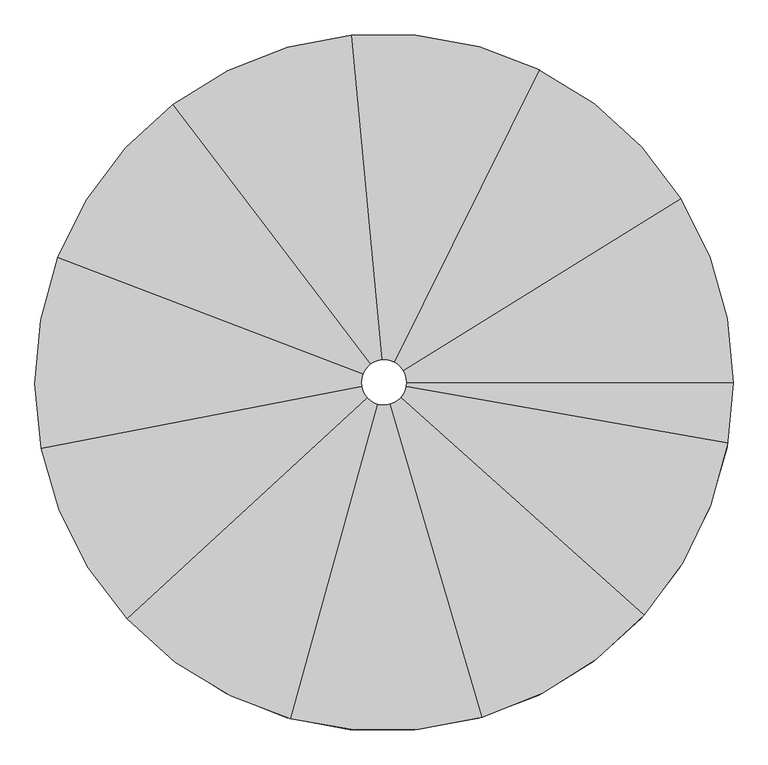
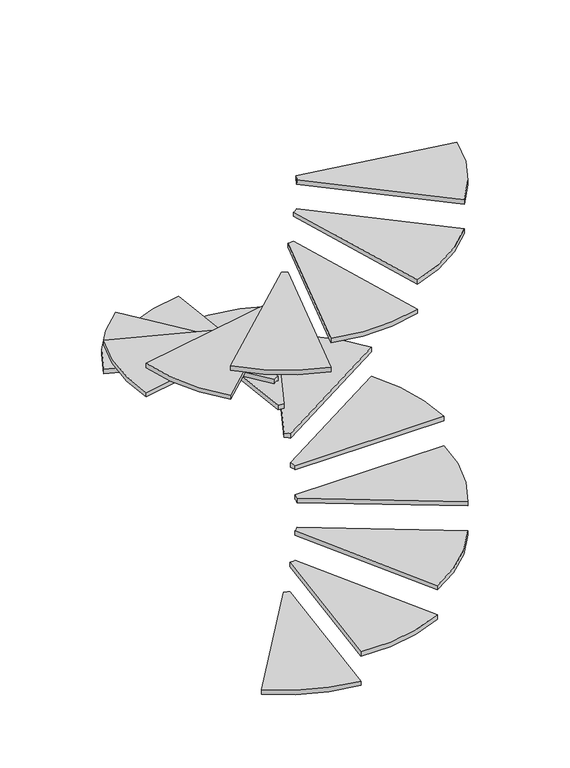
"""IFC4 building model written with IfcOpenShell, lengths in millimetres: stair flight geometry."""

from ifc_helpers import new_model, si_unit, point, frame, frame_2d, origin, place, context, project, spatial, polyline, circle_curve, trimmed, segment, composite_curve, outline, extrude, source, transform, mapped, element, save


def stair_flight_6586929f(model_context):
    return source(origin(), model_context, "Body", "SweptSolid", [
        extrude(outline(composite_curve([segment(polyline([(21449.895584, -2902.3142462), (21371.5931684, -3711.3337588)]), True, "CONTINUOUS"), segment(trimmed(circle_curve(frame_2d((21455.3703815, -2845.7487117)), 869.6298611), [point((21371.5931684, -3711.3337588))], [point((20927.7521934, -3537.0338502))], False, "CARTESIAN"), True, "CONTINUOUS"), segment(polyline([(20927.7521934, -3537.0338502), (21420.8908061, -2890.9238375)]), True, "CONTINUOUS"), segment(trimmed(circle_curve(frame_2d((21455.3703815, -2845.7487117)), 56.8298611), [point((21420.8908061, -2890.9238375))], [point((21449.895584, -2902.3142462))], True, "CARTESIAN"), True, "CONTINUOUS")], self_intersect=False)), frame((0.0, 0.0, 142.875), z_axis=(0.0, 0.0, 1.0), x_axis=(1.0, 0.0, 0.0)), (0.0, 0.0, 1.0), 25.4),
        extrude(outline(composite_curve([segment(polyline([(21480.5464095, -2896.6977129), (21840.6225241, -3625.387655)]), True, "CONTINUOUS"), segment(trimmed(circle_curve(frame_2d((21455.3703815, -2845.7487117)), 869.6298611), [point((21840.6225241, -3625.387655))], [point((21371.5931684, -3711.3337588))], False, "CARTESIAN"), True, "CONTINUOUS"), segment(polyline([(21371.5931684, -3711.3337588), (21449.895584, -2902.3142462)]), True, "CONTINUOUS"), segment(trimmed(circle_curve(frame_2d((21455.3703815, -2845.7487117)), 56.8298611), [point((21449.895584, -2902.3142462))], [point((21480.5464095, -2896.6977129))], True, "CARTESIAN"), True, "CONTINUOUS")], self_intersect=False)), frame((0.0, 0.0, 311.15), z_axis=(0.0, 0.0, 1.0), x_axis=(1.0, 0.0, 0.0)), (0.0, 0.0, 1.0), 25.4),
        extrude(outline(composite_curve([segment(polyline([(21503.6278333, -2875.7628992), (22193.8223212, -3305.0360161)]), True, "CONTINUOUS"), segment(trimmed(circle_curve(frame_2d((21455.3703815, -2845.7487117)), 869.6298611), [point((22193.8223212, -3305.0360161))], [point((21840.6225241, -3625.387655))], False, "CARTESIAN"), True, "CONTINUOUS"), segment(polyline([(21840.6225241, -3625.387655), (21480.5464095, -2896.6977129)]), True, "CONTINUOUS"), segment(trimmed(circle_curve(frame_2d((21455.3703815, -2845.7487117)), 56.8298611), [point((21480.5464095, -2896.6977129))], [point((21503.6278333, -2875.7628992))], True, "CARTESIAN"), True, "CONTINUOUS")], self_intersect=False)), frame((0.0, 0.0, 479.425), z_axis=(0.0, 0.0, 1.0), x_axis=(1.0, 0.0, 0.0)), (0.0, 0.0, 1.0), 25.4),
        extrude(outline(composite_curve([segment(polyline([(21512.2002156, -2845.8040472), (22324.9998303, -2846.5954743)]), True, "CONTINUOUS"), segment(trimmed(circle_curve(frame_2d((21455.3703815, -2845.7487117)), 869.6298611), [point((22324.9998303, -2846.5954743))], [point((22193.8223212, -3305.0360161))], False, "CARTESIAN"), True, "CONTINUOUS"), segment(polyline([(22193.8223212, -3305.0360161), (21503.6278333, -2875.7628992)]), True, "CONTINUOUS"), segment(trimmed(circle_curve(frame_2d((21455.3703815, -2845.7487117)), 56.8298611), [point((21503.6278333, -2875.7628992))], [point((21512.2002156, -2845.8040472))], True, "CARTESIAN"), True, "CONTINUOUS")], self_intersect=False)), frame((0.0, 0.0, 647.7), z_axis=(0.0, 0.0, 1.0), x_axis=(1.0, 0.0, 0.0)), (0.0, 0.0, 1.0), 25.4),
        extrude(outline(composite_curve([segment(polyline([(21503.6861917, -2815.828558), (22194.7153409, -2387.9003456)]), True, "CONTINUOUS"), segment(trimmed(circle_curve(frame_2d((21455.3703815, -2845.7487117)), 869.6298611), [point((22194.7153409, -2387.9003456))], [point((22324.9998303, -2846.5954743))], False, "CARTESIAN"), True, "CONTINUOUS"), segment(polyline([(22324.9998303, -2846.5954743), (21512.2002156, -2845.8040472)]), True, "CONTINUOUS"), segment(trimmed(circle_curve(frame_2d((21455.3703815, -2845.7487117)), 56.8298611), [point((21512.2002156, -2845.8040472))], [point((21503.6861917, -2815.828558))], True, "CARTESIAN"), True, "CONTINUOUS")], self_intersect=False)), frame((0.0, 0.0, 815.975), z_axis=(0.0, 0.0, 1.0), x_axis=(1.0, 0.0, 0.0)), (0.0, 0.0, 1.0), 25.4),
        extrude(outline(composite_curve([segment(polyline([(21480.6455803, -2794.8488351), (21842.140069, -2066.8614899)]), True, "CONTINUOUS"), segment(trimmed(circle_curve(frame_2d((21455.3703815, -2845.7487117)), 869.6298611), [point((21842.140069, -2066.8614899))], [point((22194.7153409, -2387.9003456))], False, "CARTESIAN"), True, "CONTINUOUS"), segment(polyline([(22194.7153409, -2387.9003456), (21503.6861917, -2815.828558)]), True, "CONTINUOUS"), segment(trimmed(circle_curve(frame_2d((21455.3703815, -2845.7487117)), 56.8298611), [point((21503.6861917, -2815.828558))], [point((21480.6455803, -2794.8488351))], True, "CARTESIAN"), True, "CONTINUOUS")], self_intersect=False)), frame((0.0, 0.0, 984.25), z_axis=(0.0, 0.0, 1.0), x_axis=(1.0, 0.0, 0.0)), (0.0, 0.0, 1.0), 25.4),
        extrude(outline(composite_curve([segment(polyline([(21450.0057506, -2789.1726227), (21373.2789748, -1980.0021574)]), True, "CONTINUOUS"), segment(trimmed(circle_curve(frame_2d((21455.3703815, -2845.7487117)), 869.6298611), [point((21373.2789748, -1980.0021574))], [point((21842.140069, -2066.8614899))], False, "CARTESIAN"), True, "CONTINUOUS"), segment(polyline([(21842.140069, -2066.8614899), (21480.6455803, -2794.8488351)]), True, "CONTINUOUS"), segment(trimmed(circle_curve(frame_2d((21455.3703815, -2845.7487117)), 56.8298611), [point((21480.6455803, -2794.8488351))], [point((21450.0057506, -2789.1726227))], True, "CARTESIAN"), True, "CONTINUOUS")], self_intersect=False)), frame((0.0, 0.0, 1152.525), z_axis=(0.0, 0.0, 1.0), x_axis=(1.0, 0.0, 0.0)), (0.0, 0.0, 1.0), 25.4),
        extrude(outline(composite_curve([segment(polyline([(21420.9788459, -2800.5065257), (20929.0994083, -2153.4373958)]), True, "CONTINUOUS"), segment(trimmed(circle_curve(frame_2d((21455.3703815, -2845.7487117)), 869.6298611), [point((20929.0994083, -2153.4373958))], [point((21373.2789748, -1980.0021574))], False, "CARTESIAN"), True, "CONTINUOUS"), segment(polyline([(21373.2789748, -1980.0021574), (21450.0057506, -2789.1726227)]), True, "CONTINUOUS"), segment(trimmed(circle_curve(frame_2d((21455.3703815, -2845.7487117)), 56.8298611), [point((21450.0057506, -2789.1726227))], [point((21420.9788459, -2800.5065257))], True, "CARTESIAN"), True, "CONTINUOUS")], self_intersect=False)), frame((0.0, 0.0, 1320.8), z_axis=(0.0, 0.0, 1.0), x_axis=(1.0, 0.0, 0.0)), (0.0, 0.0, 1.0), 25.4),
        extrude(outline(composite_curve([segment(polyline([(21402.292069, -2825.4429031), (20643.1479935, -2535.0223243)]), True, "CONTINUOUS"), segment(trimmed(circle_curve(frame_2d((21455.3703815, -2845.7487117)), 869.6298611), [point((20643.1479935, -2535.0223243))], [point((20929.0994083, -2153.4373958))], False, "CARTESIAN"), True, "CONTINUOUS"), segment(polyline([(20929.0994083, -2153.4373958), (21420.9788459, -2800.5065257)]), True, "CONTINUOUS"), segment(trimmed(circle_curve(frame_2d((21455.3703815, -2845.7487117)), 56.8298611), [point((21420.9788459, -2800.5065257))], [point((21402.292069, -2825.4429031))], True, "CARTESIAN"), True, "CONTINUOUS")], self_intersect=False)), frame((0.0, 0.0, 1489.075), z_axis=(0.0, 0.0, 1.0), x_axis=(1.0, 0.0, 0.0)), (0.0, 0.0, 1.0), 25.4),
        extrude(outline(composite_curve([segment(polyline([(21399.5637693, -2856.4844065), (20601.3986226, -3010.0299656)]), True, "CONTINUOUS"), segment(trimmed(circle_curve(frame_2d((21455.3703815, -2845.7487117)), 869.6298611), [point((20601.3986226, -3010.0299656))], [point((20643.1479935, -2535.0223243))], False, "CARTESIAN"), True, "CONTINUOUS"), segment(polyline([(20643.1479935, -2535.0223243), (21402.292069, -2825.4429031)]), True, "CONTINUOUS"), segment(trimmed(circle_curve(frame_2d((21455.3703815, -2845.7487117)), 56.8298611), [point((21402.292069, -2825.4429031))], [point((21399.5637693, -2856.4844065))], True, "CARTESIAN"), True, "CONTINUOUS")], self_intersect=False)), frame((0.0, 0.0, 1657.35), z_axis=(0.0, 0.0, 1.0), x_axis=(1.0, 0.0, 0.0)), (0.0, 0.0, 1.0), 25.4),
        extrude(outline(composite_curve([segment(polyline([(21413.6142347, -2884.2981257), (20816.4036234, -3435.6449546)]), True, "CONTINUOUS"), segment(trimmed(circle_curve(frame_2d((21455.3703815, -2845.7487117)), 869.6298611), [point((20816.4036234, -3435.6449546))], [point((20601.3986226, -3010.0299656))], False, "CARTESIAN"), True, "CONTINUOUS"), segment(polyline([(20601.3986226, -3010.0299656), (21399.5637693, -2856.4844065)]), True, "CONTINUOUS"), segment(trimmed(circle_curve(frame_2d((21455.3703815, -2845.7487117)), 56.8298611), [point((21399.5637693, -2856.4844065))], [point((21413.6142347, -2884.2981257))], True, "CARTESIAN"), True, "CONTINUOUS")], self_intersect=False)), frame((0.0, 0.0, 1825.625), z_axis=(0.0, 0.0, 1.0), x_axis=(1.0, 0.0, 0.0)), (0.0, 0.0, 1.0), 25.4),
        extrude(outline(composite_curve([segment(polyline([(21440.2190653, -2900.5216131), (21223.5197881, -3683.9022761)]), True, "CONTINUOUS"), segment(trimmed(circle_curve(frame_2d((21455.3703815, -2845.7487117)), 869.6298611), [point((21223.5197881, -3683.9022761))], [point((20816.4036234, -3435.6449546))], False, "CARTESIAN"), True, "CONTINUOUS"), segment(polyline([(20816.4036234, -3435.6449546), (21413.6142347, -2884.2981257)]), True, "CONTINUOUS"), segment(trimmed(circle_curve(frame_2d((21455.3703815, -2845.7487117)), 56.8298611), [point((21413.6142347, -2884.2981257))], [point((21440.2190653, -2900.5216131))], True, "CARTESIAN"), True, "CONTINUOUS")], self_intersect=False)), frame((0.0, 0.0, 1993.9), z_axis=(0.0, 0.0, 1.0), x_axis=(1.0, 0.0, 0.0)), (0.0, 0.0, 1.0), 25.4),
        extrude(outline(composite_curve([segment(polyline([(21471.3792768, -2900.2771298), (21700.3439412, -3680.1611099)]), True, "CONTINUOUS"), segment(trimmed(circle_curve(frame_2d((21455.3703815, -2845.7487117)), 869.6298611), [point((21700.3439412, -3680.1611099))], [point((21223.5197881, -3683.9022761))], False, "CARTESIAN"), True, "CONTINUOUS"), segment(polyline([(21223.5197881, -3683.9022761), (21440.2190653, -2900.5216131)]), True, "CONTINUOUS"), segment(trimmed(circle_curve(frame_2d((21455.3703815, -2845.7487117)), 56.8298611), [point((21440.2190653, -2900.5216131))], [point((21471.3792768, -2900.2771298))], True, "CARTESIAN"), True, "CONTINUOUS")], self_intersect=False)), frame((0.0, 0.0, 2162.175), z_axis=(0.0, 0.0, 1.0), x_axis=(1.0, 0.0, 0.0)), (0.0, 0.0, 1.0), 25.4),
        extrude(outline(composite_curve([segment(polyline([(21497.7262684, -2883.6381819), (22103.5145667, -3425.5462715)]), True, "CONTINUOUS"), segment(trimmed(circle_curve(frame_2d((21455.3703815, -2845.7487117)), 869.6298611), [point((22103.5145667, -3425.5462715))], [point((21700.3439412, -3680.1611099))], False, "CARTESIAN"), True, "CONTINUOUS"), segment(polyline([(21700.3439412, -3680.1611099), (21471.3792768, -2900.2771298)]), True, "CONTINUOUS"), segment(trimmed(circle_curve(frame_2d((21455.3703815, -2845.7487117)), 56.8298611), [point((21471.3792768, -2900.2771298))], [point((21497.7262684, -2883.6381819))], True, "CARTESIAN"), True, "CONTINUOUS")], self_intersect=False)), frame((0.0, 0.0, 2330.45), z_axis=(0.0, 0.0, 1.0), x_axis=(1.0, 0.0, 0.0)), (0.0, 0.0, 1.0), 25.4),
        extrude(outline(composite_curve([segment(polyline([(21511.3385776, -2855.6074205), (22311.8147515, -2996.6100265)]), True, "CONTINUOUS"), segment(trimmed(circle_curve(frame_2d((21455.3703815, -2845.7487117)), 869.6298611), [point((22311.8147515, -2996.6100265))], [point((22103.5145667, -3425.5462715))], False, "CARTESIAN"), True, "CONTINUOUS"), segment(polyline([(22103.5145667, -3425.5462715), (21497.7262684, -2883.6381819)]), True, "CONTINUOUS"), segment(trimmed(circle_curve(frame_2d((21455.3703815, -2845.7487117)), 56.8298611), [point((21497.7262684, -2883.6381819))], [point((21511.3385776, -2855.6074205))], True, "CARTESIAN"), True, "CONTINUOUS")], self_intersect=False)), frame((0.0, 0.0, 2498.725), z_axis=(0.0, 0.0, 1.0), x_axis=(1.0, 0.0, 0.0)), (0.0, 0.0, 1.0), 25.4),
    ])


if __name__ == "__main__":
    model = new_model("IFC4")
    model_context = context("Model", 3, world=origin())
    ifc_project = project(units=[si_unit("LENGTHUNIT", "METRE", prefix="MILLI")], contexts=[model_context])
    site = spatial("IfcSite", under=ifc_project)
    building = spatial("IfcBuilding", under=site)
    placement = place(None, origin())
    stair_flight_shape = stair_flight_6586929f(model_context)
    element("IfcStairFlight", 1, at=placement, inside=building, context=model_context, shape_type="MappedRepresentation", body=[
        mapped(stair_flight_shape, transform((0.0, 0.0, 0.0), x_axis=(1.0, 0.0, 0.0), y_axis=(0.0, 1.0, 0.0), z_axis=(0.0, 0.0, 1.0))),
    ])
    save(model, "model.ifc")

# Revit data of these elements
# Element 1 (IfcStairFlight)
#   Materials on its faces: "accent 2"
# Materials
#   "accent 2": class "Wood", colour RGB 80 80 80, transparency 0, Description = "Wood framing, thermal airspace", Cost = 0
